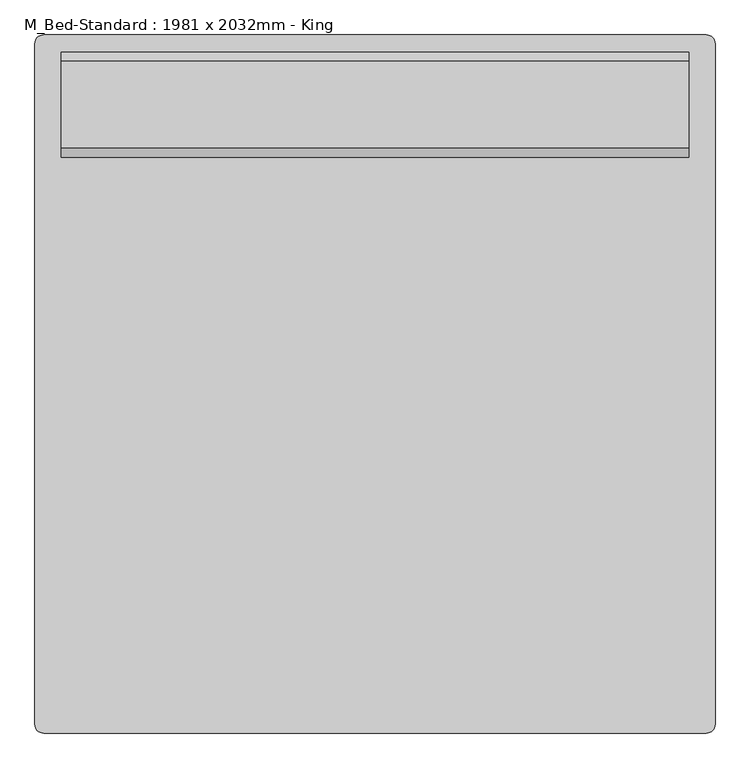
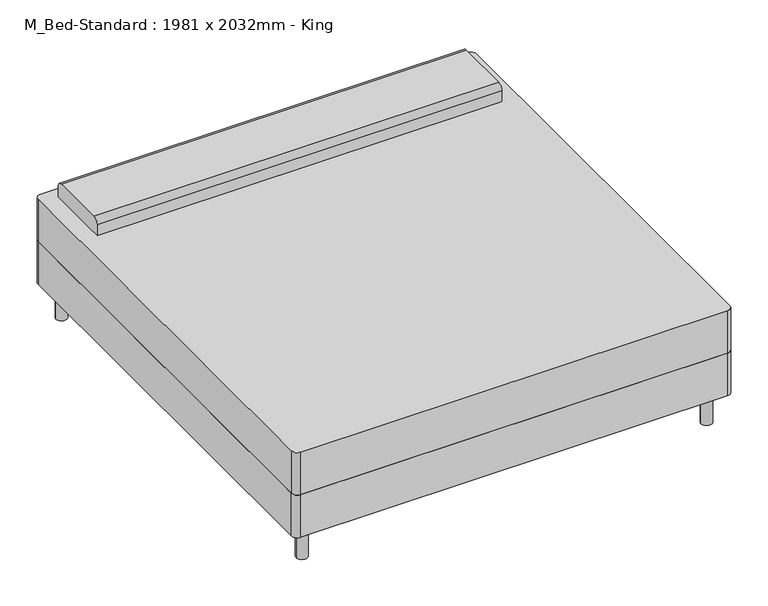
"""IFC4 building model written with IfcOpenShell, lengths in millimetres: furniture geometry, M_Bed-Standard : 1981 x 2032mm - King."""

from ifc_helpers import new_model, si_unit, point, frame, frame_2d, origin, origin_with_axes, place, context, project, spatial, polyline, circle_curve, trimmed, segment, composite_curve, outline, extrude, source, transform, mapped, element, save


def m_bed_standard_1981_x_2032mm_king_79a78f5c(model_context):
    return source(origin(), model_context, "Body", "SweptSolid", [
        extrude(outline(composite_curve([segment(polyline([(-719.0114754, -1036.195082), (-719.0114754, 945.004918)]), True, "CONTINUOUS"), segment(trimmed(circle_curve(frame_2d((-693.6114754, 945.004918)), 25.4), [point((-719.0114754, 945.004918))], [point((-693.6114754, 970.404918))], False, "CARTESIAN"), True, "CONTINUOUS"), segment(polyline([(-693.6114754, 970.404918), (1236.5885246, 970.404918)]), True, "CONTINUOUS"), segment(trimmed(circle_curve(frame_2d((1236.5885246, 945.004918)), 25.4), [point((1236.5885246, 970.404918))], [point((1261.9885246, 945.004918))], False, "CARTESIAN"), True, "CONTINUOUS"), segment(polyline([(1261.9885246, 945.004918), (1261.9885246, -1036.195082)]), True, "CONTINUOUS"), segment(trimmed(circle_curve(frame_2d((1236.5885246, -1036.195082)), 25.4), [point((1261.9885246, -1036.195082))], [point((1236.5885246, -1061.595082))], False, "CARTESIAN"), True, "CONTINUOUS"), segment(polyline([(1236.5885246, -1061.595082), (-693.6114754, -1061.595082)]), True, "CONTINUOUS"), segment(trimmed(circle_curve(frame_2d((-693.6114754, -1036.195082)), 25.4), [point((-693.6114754, -1061.595082))], [point((-719.0114754, -1036.195082))], False, "CARTESIAN"), True, "CONTINUOUS")], self_intersect=False)), frame((0.0, 0.0, 152.4), z_axis=(0.0, 0.0, 1.0), x_axis=(1.0, 0.0, 0.0)), (0.0, 0.0, 1.0), 203.2),
        extrude(outline(composite_curve([segment(polyline([(614.804918, 558.8), (614.804918, 609.6)]), True, "CONTINUOUS"), segment(trimmed(circle_curve(frame_2d((640.204918, 609.6)), 25.4), [point((614.804918, 609.6))], [point((640.204918, 635.0))], False, "CARTESIAN"), True, "CONTINUOUS"), segment(polyline([(640.204918, 635.0), (894.204918, 635.0)]), True, "CONTINUOUS"), segment(trimmed(circle_curve(frame_2d((894.204918, 609.6)), 25.4), [point((894.204918, 635.0))], [point((919.604918, 609.6))], False, "CARTESIAN"), True, "CONTINUOUS"), segment(polyline([(919.604918, 609.6), (919.604918, 558.8), (614.804918, 558.8)]), True, "CONTINUOUS")], self_intersect=False)), frame((-642.8114754, 0.0, 0.0), z_axis=(1.0, 0.0, 0.0), x_axis=(0.0, 1.0, 0.0)), (0.0, 0.0, 1.0), 1828.6),
        extrude(outline(composite_curve([segment(trimmed(circle_curve(frame_2d((-642.8114754, 894.204918)), 25.4), [point((-668.2114754, 894.204918))], [point((-617.4114754, 894.204918))], False, "CARTESIAN"), True, "CONTINUOUS"), segment(trimmed(circle_curve(frame_2d((-642.8114754, 894.204918)), 25.4), [point((-617.4114754, 894.204918))], [point((-668.2114754, 894.204918))], False, "CARTESIAN"), True, "CONTINUOUS")], self_intersect=False)), origin_with_axes(), (0.0, 0.0, 1.0), 152.4),
        extrude(outline(composite_curve([segment(trimmed(circle_curve(frame_2d((1185.7885246, 894.204918)), 25.4), [point((1160.3885246, 894.204918))], [point((1211.1885246, 894.204918))], False, "CARTESIAN"), True, "CONTINUOUS"), segment(trimmed(circle_curve(frame_2d((1185.7885246, 894.204918)), 25.4), [point((1211.1885246, 894.204918))], [point((1160.3885246, 894.204918))], False, "CARTESIAN"), True, "CONTINUOUS")], self_intersect=False)), origin_with_axes(), (0.0, 0.0, 1.0), 152.4),
        extrude(outline(composite_curve([segment(trimmed(circle_curve(frame_2d((1185.7885246, -985.395082)), 25.4), [point((1160.3885246, -985.395082))], [point((1211.1885246, -985.395082))], False, "CARTESIAN"), True, "CONTINUOUS"), segment(trimmed(circle_curve(frame_2d((1185.7885246, -985.395082)), 25.4), [point((1211.1885246, -985.395082))], [point((1160.3885246, -985.395082))], False, "CARTESIAN"), True, "CONTINUOUS")], self_intersect=False)), origin_with_axes(), (0.0, 0.0, 1.0), 152.4),
        extrude(outline(composite_curve([segment(trimmed(circle_curve(frame_2d((-642.8114754, -985.395082)), 25.4), [point((-668.2114754, -985.395082))], [point((-617.4114754, -985.395082))], False, "CARTESIAN"), True, "CONTINUOUS"), segment(trimmed(circle_curve(frame_2d((-642.8114754, -985.395082)), 25.4), [point((-617.4114754, -985.395082))], [point((-668.2114754, -985.395082))], False, "CARTESIAN"), True, "CONTINUOUS")], self_intersect=False)), origin_with_axes(), (0.0, 0.0, 1.0), 152.4),
        extrude(outline(composite_curve([segment(polyline([(-693.6114754, 970.404918), (1236.5885246, 970.404918)]), True, "CONTINUOUS"), segment(trimmed(circle_curve(frame_2d((1236.5885246, 945.004918)), 25.4), [point((1236.5885246, 970.404918))], [point((1261.9885246, 945.004918))], False, "CARTESIAN"), True, "CONTINUOUS"), segment(polyline([(1261.9885246, 945.004918), (1261.9885246, -1036.195082)]), True, "CONTINUOUS"), segment(trimmed(circle_curve(frame_2d((1236.5885246, -1036.195082)), 25.4), [point((1261.9885246, -1036.195082))], [point((1236.5885246, -1061.595082))], False, "CARTESIAN"), True, "CONTINUOUS"), segment(polyline([(1236.5885246, -1061.595082), (-693.6114754, -1061.595082)]), True, "CONTINUOUS"), segment(trimmed(circle_curve(frame_2d((-693.6114754, -1036.195082)), 25.4), [point((-693.6114754, -1061.595082))], [point((-719.0114754, -1036.195082))], False, "CARTESIAN"), True, "CONTINUOUS"), segment(polyline([(-719.0114754, -1036.195082), (-719.0114754, 945.004918)]), True, "CONTINUOUS"), segment(trimmed(circle_curve(frame_2d((-693.6114754, 945.004918)), 25.4), [point((-719.0114754, 945.004918))], [point((-693.6114754, 970.404918))], False, "CARTESIAN"), True, "CONTINUOUS")], self_intersect=False)), frame((0.0, 0.0, 355.6), z_axis=(0.0, 0.0, 1.0), x_axis=(1.0, 0.0, 0.0)), (0.0, 0.0, 1.0), 203.2),
    ])


if __name__ == "__main__":
    model = new_model("IFC4")
    model_context = context("Model", 3, world=origin())
    ifc_project = project(units=[si_unit("LENGTHUNIT", "METRE", prefix="MILLI")], contexts=[model_context])
    site = spatial("IfcSite", under=ifc_project)
    building = spatial("IfcBuilding", under=site)
    placement = place(None, origin())
    m_bed_standard_1981_x_2032mm_king_shape = m_bed_standard_1981_x_2032mm_king_79a78f5c(model_context)
    element("IfcFurniture", 1, ObjectType="M_Bed-Standard : 1981 x 2032mm - King", at=placement, inside=building, context=model_context, shape_type="MappedRepresentation", body=[
        mapped(m_bed_standard_1981_x_2032mm_king_shape, transform((0.0, 0.0, 0.0), x_axis=(1.0, 0.0, 0.0), y_axis=(0.0, 1.0, 0.0), z_axis=(0.0, 0.0, 1.0))),
    ])
    save(model, "model.ifc")

# Revit data of these elements
# Type "M_Bed-Standard : 1981 x 2032mm - King"
#   Manufacturer = "Manufacturer"
#   AccessibilityPerformance = "AccessibilityPerformance"
#   CodePerformance = "CodePerformance"
#   Area = "Area"
#   Color = "Color"
#   Constituents = "Constituents"
#   Features = "Features"
#   Finish = "Finish"
#   Grade = "Grade"
#   Material = "Material"
#   ModelReference = "ModelReference"
#   NominalHeight = "NominalHeight"
#   NominalLength = "NominalLength"
#   NominalWidth = "NominalWidth"
#   ProductionYear = "ProductionYear"
#   Reference = "Reference"
#   Shape = "Shape"
#   Size = "Size"
#   SustainabilityPerformance = "SustainabilityPerformance"
#   WarrantyDescription = "WarrantyDescription"
#   WarrantyDurationLabor = "WarrantyDurationLabor"
#   WarrantyDurationParts = "WarrantyDurationParts"
#   WarrantyGuarantorLabor = "WarrantyGuarantorLabor"
#   WarrantyGuarantorParts = "WarrantyGuarantorParts"
#   ExpectedLife = "ExpectedLife"
#   ReplacementCost = "ReplacementCost"
#   AssetAccountingType = "NONFIXED"
#   ModelLabel = "ModelLabel"
#   Length = 2.032 m
#   Width = 1.981 m
#   Leg Material = Metal - Chrome
#   Mattress Material = Textile - White
# Element 1 (IfcFurniture, "M_Bed-Standard : 1981 x 2032mm - King")
#   Materials on its faces: "Textile - White", "Metal - Chrome"
# Materials
#   "Metal - Chrome": class "Metal", colour RGB 17 17 17, transparency 0
#   "Textile - White": class "Fabric", colour RGB 247 247 239, transparency 0
